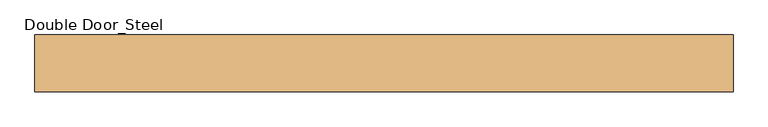
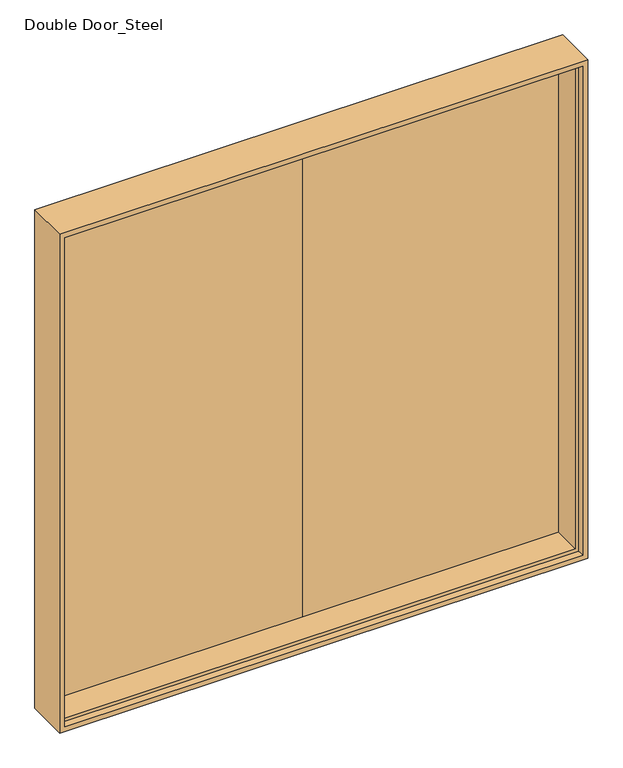
"""IFC4 building model written with IfcOpenShell, lengths in millimetres: door geometry, Double Door_Steel : H_DR_AR B12_Door_Double_W2100xH2280_No FR_SD-4."""

from ifc_helpers import new_model, si_unit, frame, origin, place, context, project, spatial, polyline, outline, extrude, faceted_brep, source, transform, mapped, element, save


def double_door_steel_886c32a2(model_context):
    return source(origin(), model_context, "Body", "SolidModel", [
        faceted_brep([(1535.0, -125.0, 3065.0), (1535.0, 125.0, 3065.0), (-1535.0, 125.0, 3065.0), (-1535.0, -125.0, 3065.0), (1485.0, 85.0, 3015.0), (1485.0, -85.0, 3015.0), (-1485.0, -85.0, 3015.0), (-1485.0, 85.0, 3015.0), (1505.0, 125.0, 3035.0), (1505.0, 85.0, 3035.0), (-1505.0, 85.0, 3035.0), (-1505.0, 125.0, 3035.0), (-1535.0, 125.0, 0.0), (-1535.0, -125.0, 0.0), (-1485.0, -85.0, 50.0), (-1485.0, 85.0, 50.0), (-1505.0, 85.0, 30.0), (-1505.0, 125.0, 30.0), (1535.0, 125.0, 0.0), (1505.0, 125.0, 30.0), (1535.0, -125.0, 0.0), (1505.0, -125.0, 30.0), (-1505.0, -125.0, 30.0), (-1505.0, -125.0, 3035.0), (1505.0, -125.0, 3035.0), (1485.0, -85.0, 50.0), (1485.0, 85.0, 50.0), (1505.0, 85.0, 30.0), (1505.0, -85.0, 30.0), (1505.0, -85.0, 3035.0), (-1505.0, -85.0, 3035.0), (-1505.0, -85.0, 30.0)], [[[0, 1, 2, 3]], [[4, 5, 6, 7]], [[8, 9, 10, 11]], [[3, 2, 12, 13]], [[7, 6, 14, 15]], [[11, 10, 16, 17]], [[18, 12, 2, 1], [8, 11, 17, 19]], [[13, 12, 18, 20]], [[0, 3, 13, 20], [21, 22, 23, 24]], [[15, 14, 25, 26]], [[27, 16, 10, 9], [4, 7, 15, 26]], [[17, 16, 27, 19]], [[20, 18, 1, 0]], [[26, 25, 5, 4]], [[19, 27, 9, 8]], [[28, 21, 24, 29]], [[29, 24, 23, 30]], [[30, 23, 22, 31]], [[30, 31, 28, 29], [5, 25, 14, 6]], [[31, 22, 21, 28]]]),
        extrude(outline(polyline([(1505.0, 85.0), (0.0, 85.0), (0.0, 125.0), (1505.0, 125.0), (1505.0, 85.0)])), frame((0.0, 0.0, 30.0), z_axis=(0.0, 0.0, 1.0), x_axis=(1.0, 0.0, 0.0)), (0.0, 0.0, 1.0), 3005.0),
        extrude(outline(polyline([(0.0, 85.0), (-1505.0, 85.0), (-1505.0, 125.0), (0.0, 125.0), (0.0, 85.0)])), frame((0.0, 0.0, 30.0), z_axis=(0.0, 0.0, 1.0), x_axis=(1.0, 0.0, 0.0)), (0.0, 0.0, 1.0), 3005.0),
    ])


if __name__ == "__main__":
    model = new_model("IFC4")
    model_context = context("Model", 3, world=origin())
    ifc_project = project(units=[si_unit("LENGTHUNIT", "METRE", prefix="MILLI")], contexts=[model_context])
    site = spatial("IfcSite", under=ifc_project)
    building = spatial("IfcBuilding", under=site)
    placement = place(None, origin())
    double_door_steel_shape = double_door_steel_886c32a2(model_context)
    element("IfcDoor", 1, ObjectType="Double Door_Steel : H_DR_AR B12_Door_Double_W2100xH2280_No FR_SD-4", at=placement, inside=building, context=model_context, shape_type="MappedRepresentation", body=[
        mapped(double_door_steel_shape, transform((0.0, 0.0, 0.0), x_axis=(1.0, 0.0, 0.0), y_axis=(0.0, 1.0, 0.0), z_axis=(0.0, 0.0, 1.0))),
    ])
    save(model, "model.ifc")

# Revit data of these elements
# Type "Double Door_Steel : H_DR_AR B12_Door_Double_W2100xH2280_No FR_SD-4"
#   Type Mark = "440"
#   프레임 = ""
#   철물 = ""
#   유리/마감 = ""
#   위치/개소 = ""
#   부호 = ""
#   문번호 = ""
#   문기호 = "SD-4"
#   Analytic Construction = "<None>"
#   Door Width = 1505 mm
#   Height = 3080 mm
#   Width = 3100 mm
#   Define Thermal Properties by = 1
#   문 틀 = none
#   문 = none
#   Function = (empty or 0)
#   Assembly Code = ""
#   Wall Closure = (empty or 0)
